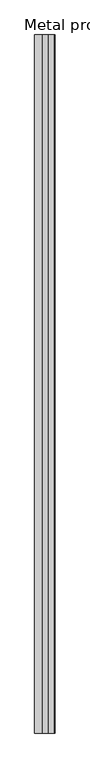
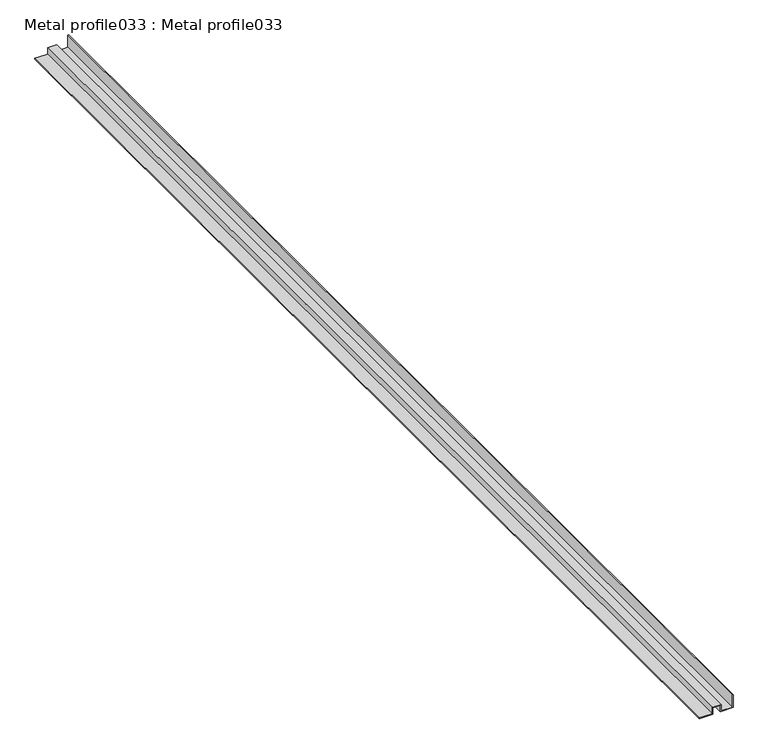
"""IFC4 building model written with IfcOpenShell, lengths in millimetres: proxy geometry, Metal profile033 : Metal profile033."""

from ifc_helpers import new_model, si_unit, frame, origin, place, context, project, spatial, polyline, outline, extrude, source, transform, mapped, element, save


def metal_profile033_metal_profile033_c745fb2b(model_context):
    return source(origin(), model_context, "Body", "SweptSolid", [
        extrude(outline(polyline([(39542.6175708, -9269.4987353), (39566.4183323, -9269.4987353), (39566.4183323, -9270.7787353), (39543.8975708, -9270.7787353), (39543.8975708, -9290.4437353), (39555.3275708, -9290.4437353), (39555.3275708, -9305.7037353), (39543.8975708, -9305.7037353), (39543.8975708, -9328.1369192), (39542.6175708, -9328.1369192), (39542.6175708, -9304.4237353), (39554.0475708, -9304.4237353), (39554.0475708, -9291.7237353), (39542.6175708, -9291.7237353), (39542.6175708, -9269.4987353)])), frame((0.0, 7982.1531721, 0.0), z_axis=(0.0, 1.0, 0.0), x_axis=(0.0, 0.0, 1.0)), (0.0, 0.0, 1.0), 2000.0),
    ])


if __name__ == "__main__":
    model = new_model("IFC4")
    model_context = context("Model", 3, world=origin())
    ifc_project = project(units=[si_unit("LENGTHUNIT", "METRE", prefix="MILLI")], contexts=[model_context])
    site = spatial("IfcSite", under=ifc_project)
    building = spatial("IfcBuilding", under=site)
    placement = place(None, origin())
    metal_profile033_metal_profile033_shape = metal_profile033_metal_profile033_c745fb2b(model_context)
    element("IfcBuildingElementProxy", 1, Name="Metal profile033 : Metal profile033", ObjectType="Metal profile033 : Metal profile033", at=placement, inside=building, context=model_context, shape_type="MappedRepresentation", body=[
        mapped(metal_profile033_metal_profile033_shape, transform((0.0, 0.0, 0.0), x_axis=(1.0, 0.0, 0.0), y_axis=(0.0, 1.0, 0.0), z_axis=(0.0, 0.0, 1.0))),
    ])
    save(model, "model.ifc")

# Revit data of these elements
# Type "Metal profile033 : Metal profile033"
#   NameOverride = "Metal profile033"
# Element 1 (IfcBuildingElementProxy, "Metal profile033 : Metal profile033")
#   Materials on its faces: "16 GA. COPPER SOFFIT DRIP SCREED"
# Materials
#   "16 GA. COPPER SOFFIT DRIP SCREED": class "Unassigned", colour RGB 255 217 0, transparency 0
